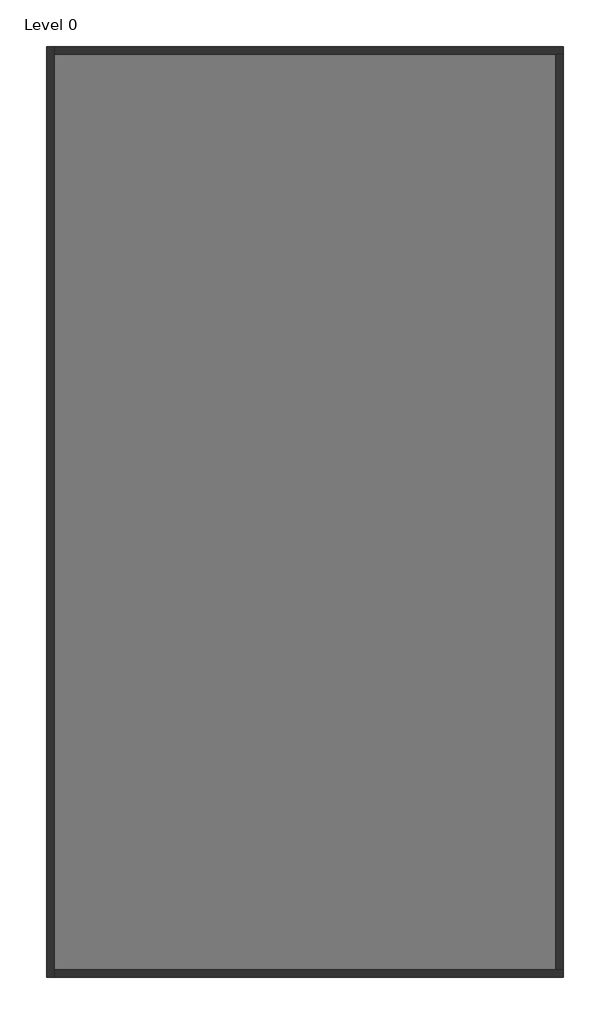
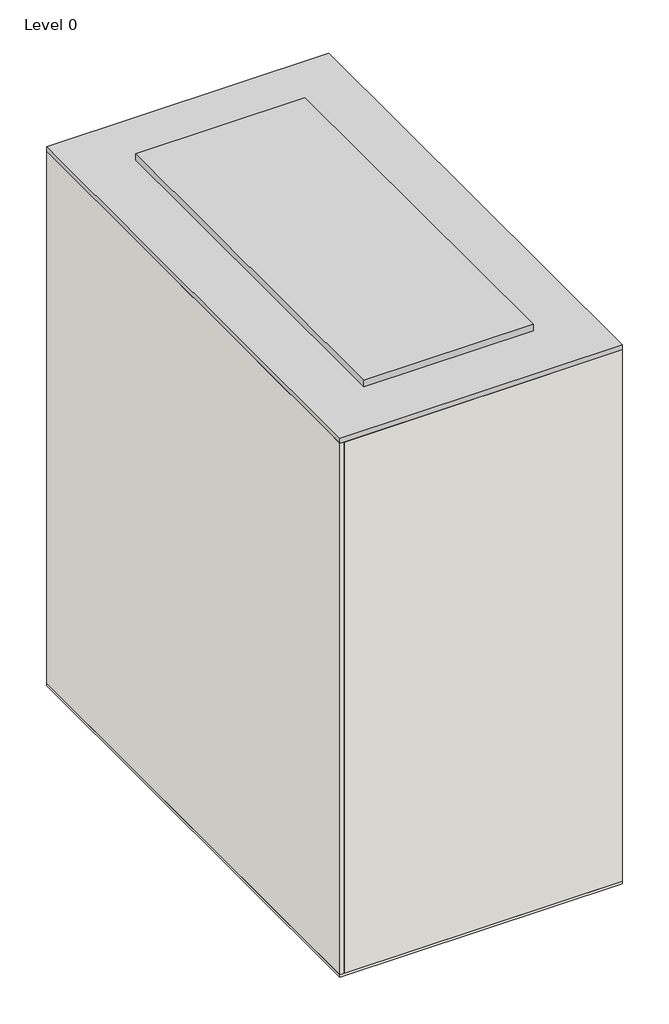
# One storey: 4 walls, 1 proxy, 1 slab.
"""IFC4 building model written with IfcOpenShell, lengths in millimetres."""

import ifcopenshell
import ifcopenshell.guid

model = None  # the IFC model being written
_history = None  # IfcOwnerHistory: only IFC2X3 demands one
_inside = {}  # id of a spatial element -> (the spatial element, [elements in it])
_under = {}  # id of a project, library or spatial element -> (it, [spatial elements below it])
_declared = {}  # id of a project -> (the project, [libraries it declares])
_typed = {}  # id of a type object -> (the type object, [elements of that type])
_made_of = {}  # id of a material, layer set ... -> (it, [elements and type objects made of it])


def new_model(schema):
    """Start an empty IFC model of exactly this schema.

    Asked for "IFC4X3", IfcOpenShell would pick the latest addendum, in which some entities
    have other attributes; the version numbers below select the first issue.
    IFC2X3 requires an IfcOwnerHistory on every rooted entity: one is made here for all.
    """
    global model, _history
    if schema == "IFC4X3":
        model = ifcopenshell.file(schema_version=(4, 3, 0, 0))
    else:
        model = ifcopenshell.file(schema=schema)
    _inside.clear()
    _under.clear()
    _declared.clear()
    _typed.clear()
    _made_of.clear()
    _history = None
    if model.schema == "IFC2X3":
        org = make("IfcOrganization", Name="unknown")
        user = make(
            "IfcPersonAndOrganization",
            ThePerson=make("IfcPerson", FamilyName="unknown"),
            TheOrganization=org,
        )
        app = make(
            "IfcApplication",
            ApplicationDeveloper=org,
            Version="unknown",
            ApplicationFullName="unknown",
            ApplicationIdentifier="unknown",
        )
        _history = make(
            "IfcOwnerHistory",
            OwningUser=user,
            OwningApplication=app,
            ChangeAction="ADDED",
            CreationDate=0,
        )
    return model


def make(cls, **values):
    """One entity of the class cls with the attributes given. An attribute that is None is left unset."""
    return model.create_entity(
        cls, **{name: value for name, value in values.items() if value is not None}
    )


def rooted(cls, **values):
    """An entity with a GlobalId (a new one), such as an element, a storey or a relation."""
    return make(cls, GlobalId=ifcopenshell.guid.new(), OwnerHistory=_history, **values)


def si_unit(unit_type, name, prefix=None):
    """IfcSIUnit, for example si_unit("LENGTHUNIT", "METRE", prefix="MILLI")."""
    return make("IfcSIUnit", UnitType=unit_type, Prefix=prefix, Name=name)


def assignment(units):
    """IfcUnitAssignment: the units of a project."""
    return None if units is None else make("IfcUnitAssignment", Units=units)


def point(xyz):
    """IfcCartesianPoint."""
    return None if xyz is None else make("IfcCartesianPoint", Coordinates=xyz)


def direction(xyz):
    """IfcDirection."""
    return None if xyz is None else make("IfcDirection", DirectionRatios=xyz)


def frame(location, z_axis=None, x_axis=None):
    """IfcAxis2Placement3D, a coordinate frame: its origin and axes. An axis left out is left unset."""
    return make(
        "IfcAxis2Placement3D",
        Location=point(location),
        Axis=direction(z_axis),
        RefDirection=direction(x_axis),
    )


def origin():
    """The frame at (0, 0, 0) with its axes left unset."""
    return frame((0.0, 0.0, 0.0))


def origin_with_axes():
    """The frame at (0, 0, 0) with the z axis (0, 0, 1) and the x axis (1, 0, 0) written out."""
    return frame((0.0, 0.0, 0.0), z_axis=(0.0, 0.0, 1.0), x_axis=(1.0, 0.0, 0.0))


def place(relative_to, where):
    """IfcLocalPlacement: puts the frame where relative to a parent placement (None: the world)."""
    return make(
        "IfcLocalPlacement", PlacementRelTo=relative_to, RelativePlacement=where
    )


def context(
    kind, dimensions, precision=None, world=None, true_north=None, identifier=None
):
    """IfcGeometricRepresentationContext, for example the 3D "Model" context."""
    return make(
        "IfcGeometricRepresentationContext",
        ContextIdentifier=identifier,
        ContextType=kind,
        CoordinateSpaceDimension=dimensions,
        Precision=precision,
        WorldCoordinateSystem=world,
        TrueNorth=true_north,
    )


def project(units=None, contexts=None):
    """IfcProject with its units and contexts."""
    return rooted(
        "IfcProject",
        Name="project",
        RepresentationContexts=contexts,
        UnitsInContext=assignment(units),
    )


def spatial(cls, under=None, at=None, **own):
    """A site, building, storey or space (cls), placed at a placement, below another one or the project."""
    s = rooted(cls, ObjectPlacement=at, **own)
    if under is not None:
        _under.setdefault(under.id(), (under, []))[1].append(s)
    return s


def polyline(points):
    """IfcPolyline through the points."""
    return make("IfcPolyline", Points=[point(p) for p in points])


def outline(outer, holes=None, kind="AREA"):
    """IfcArbitraryClosedProfileDef: a profile drawn as a closed curve; with holes, ...WithVoids."""
    if holes is None:
        return make("IfcArbitraryClosedProfileDef", ProfileType=kind, OuterCurve=outer)
    return make(
        "IfcArbitraryProfileDefWithVoids",
        ProfileType=kind,
        OuterCurve=outer,
        InnerCurves=holes,
    )


def extrude(swept, where, along, depth):
    """IfcExtrudedAreaSolid: the profile swept, set in the frame where, extruded along a direction by depth."""
    return make(
        "IfcExtrudedAreaSolid",
        SweptArea=swept,
        Position=where,
        ExtrudedDirection=direction(along),
        Depth=depth,
    )


def faces_of(points, faces, orient=None, outer=None):
    """IfcFace entities. A face is a list of loops; a loop is a list of indices into points, from 0.

    orient and outer hold one flag for each loop. By default every Orientation is true, the
    first loop of a face is its IfcFaceOuterBound and the others are IfcFaceBound.
    """
    made = []
    for i, loops in enumerate(faces):
        bounds = []
        for j, loop in enumerate(loops):
            is_outer = j == 0 if outer is None else outer[i][j]
            bounds.append(
                make(
                    "IfcFaceOuterBound" if is_outer else "IfcFaceBound",
                    Bound=make("IfcPolyLoop", Polygon=[points[k] for k in loop]),
                    Orientation=True if orient is None else orient[i][j],
                )
            )
        made.append(make("IfcFace", Bounds=bounds))
    return made


def faceted_brep(points, faces, orient=None, outer=None, voids=None):
    """IfcFacetedBrep: a solid bounded by flat faces; with voids (closed shells), ...WithVoids."""
    shared = [point(p) for p in points]
    hull = make("IfcClosedShell", CfsFaces=faces_of(shared, faces, orient, outer))
    if voids is None:
        return make("IfcFacetedBrep", Outer=hull)
    return make(
        "IfcFacetedBrepWithVoids",
        Outer=hull,
        Voids=[
            make(cls, CfsFaces=faces_of(shared, fs, o, b)) for cls, fs, o, b in voids
        ],
    )


def shape(context_of_items, identifier, shape_type, items):
    """IfcShapeRepresentation: the items that make up one representation, for example the "Body"."""
    return make(
        "IfcShapeRepresentation",
        ContextOfItems=context_of_items,
        RepresentationIdentifier=identifier,
        RepresentationType=shape_type,
        Items=items,
    )


def made_of(thing, what):
    """Note that an element or type object is made of a material, layer set ...; save() writes the relation."""
    if what is not None:
        _made_of.setdefault(what.id(), (what, []))[1].append(thing)
    return thing


def element(
    cls,
    number,
    at=None,
    inside=None,
    cuts=None,
    type_object=None,
    material=None,
    context=None,
    identifier="Body",
    shape_type=None,
    held_by="IfcProductDefinitionShape",
    body=None,
    shapes=None,
    **own,
):
    """One element of the class cls, such as IfcWall. Its Tag is "e" and its number.

    at: its placement. inside: the storey or other place that contains it. cuts: it is an
    opening in that element (IfcRelVoidsElement). A single representation is given by context,
    identifier, shape_type and body (its items); several are given by shapes. held_by: the class
    of the entity that holds the representations. save() writes the other relations.
    """
    e = rooted(cls, Tag="e%d" % number, ObjectPlacement=at, **own)
    if body is not None:
        shapes = [shape(context, identifier, shape_type, body)]
    if shapes is not None:
        e.Representation = make(held_by, Representations=shapes)
    if inside is not None:
        _inside.setdefault(inside.id(), (inside, []))[1].append(e)
    if cuts is not None:
        rooted(
            "IfcRelVoidsElement", RelatingBuildingElement=cuts, RelatedOpeningElement=e
        )
    if type_object is not None:
        _typed.setdefault(type_object.id(), (type_object, []))[1].append(e)
    return made_of(e, material)


def aggregate(whole, parts):
    """IfcRelAggregates: a whole, such as a stair, and the parts it consists of."""
    return rooted("IfcRelAggregates", RelatingObject=whole, RelatedObjects=parts)


def save(model, path):
    """Write the relations noted so far, then the file.

    IfcRelAggregates (storeys below a building ...), IfcRelContainedInSpatialStructure (elements
    in a storey), IfcRelDefinesByType, IfcRelAssociatesMaterial and IfcRelDeclares: one each for
    every whole, place, type object, material and project.
    """
    for whole, parts in _under.values():
        aggregate(whole, parts)
    for where, things in _inside.values():
        rooted(
            "IfcRelContainedInSpatialStructure",
            RelatedElements=things,
            RelatingStructure=where,
        )
    for kind, things in _typed.values():
        rooted("IfcRelDefinesByType", RelatedObjects=things, RelatingType=kind)
    for what, things in _made_of.values():
        rooted("IfcRelAssociatesMaterial", RelatedObjects=things, RelatingMaterial=what)
    for by, libraries in _declared.values():
        rooted("IfcRelDeclares", RelatingContext=by, RelatedDefinitions=libraries)
    model.write(path)


model = new_model("IFC4")

# Units and contexts
model_context = context("Model", 3, world=origin())
ifc_project = project(units=[si_unit("LENGTHUNIT", "METRE", prefix="MILLI")], contexts=[model_context])

# Site, building, storey
site = spatial("IfcSite", under=ifc_project)
building = spatial("IfcBuilding", under=site)
storey = spatial("IfcBuildingStorey", under=building, Name="Level 0", Elevation=100.0)

# Proxy
placement = place(None, origin())
element("IfcBuildingElementProxy", 1, Name="LowUrbanDensityBuilding : LowUrbanDensityBuilding", ObjectType="LowUrbanDensityBuilding : LowUrbanDensityBuilding", at=placement, inside=storey, context=model_context, shape_type="SweptSolid", body=[
    extrude(outline(polyline([(7325.2659446, 3676.2074539), (7325.2659446, -14323.7925461), (-2674.7340554, -14323.7925461), (-2674.7340554, 3676.2074539), (7325.2659446, 3676.2074539)])), origin_with_axes(), (0.0, 0.0, 1.0), 20200.0),
    extrude(outline(polyline([(5325.2659446, 1676.2074539), (5325.2659446, -12323.7925461), (-674.7340554, -12323.7925461), (-674.7340554, 1676.2074539), (5325.2659446, 1676.2074539)])), frame((0.0, 0.0, 20200.0), z_axis=(0.0, 0.0, 1.0), x_axis=(1.0, 0.0, 0.0)), (0.0, 0.0, 1.0), 245.0),
])

# Slab
element("IfcSlab", 2, ObjectType="Floor-Concrete_100Con", at=placement, inside=storey, context=model_context, shape_type="SweptSolid", body=[
    extrude(outline(polyline([(7325.2659446, 3676.2074539), (7325.2659446, -14323.7925461), (-2674.7340554, -14323.7925461), (-2674.7340554, 3676.2074539), (7325.2659446, 3676.2074539)])), origin_with_axes(), (0.0, 0.0, 1.0), 100.0),
])

# Walls
element("IfcWall", 3, ObjectType="Wall-Ext_25Rdr-100Blk-19P", at=placement, inside=storey, context=model_context, shape_type="Brep", body=[
    faceted_brep([(-2674.7340554, 3676.2074539, 100.0), (-2674.7340554, -14323.7925461, 100.0), (-2674.7340554, -14323.7925461, 20000.0), (-2674.7340554, 3676.2074539, 20000.0), (-2530.4340554, 3676.2074539, 100.0), (-2530.4340554, 3676.2074539, 20000.0), (-2530.4340554, 3531.9074539, 20000.0), (-2530.4340554, -14179.4925461, 20000.0), (-2530.4340554, -14323.7925461, 20000.0), (-2530.4340554, -14323.7925461, 100.0), (-2530.4340554, -14179.4925461, 100.0), (-2530.4340554, 3531.9074539, 100.0)], [[[0, 1, 2, 3]], [[4, 5, 6, 7, 8, 9, 10, 11]], [[1, 0, 4, 11, 10, 9]], [[3, 2, 8, 7, 6, 5]], [[2, 1, 9, 8]], [[0, 3, 5, 4]]]),
])
element("IfcWall", 4, ObjectType="Wall-Ext_25Rdr-100Blk-19P", at=placement, inside=storey, context=model_context, shape_type="Brep", body=[
    faceted_brep([(-2530.4340554, -14323.7925461, 100.0), (7325.2659446, -14323.7925461, 100.0), (7325.2659446, -14323.7925461, 20000.0), (-2530.4340554, -14323.7925461, 20000.0), (-2530.4340554, -14179.4925461, 100.0), (-2530.4340554, -14179.4925461, 20000.0), (7180.9659446, -14179.4925461, 20000.0), (7325.2659446, -14179.4925461, 20000.0), (7325.2659446, -14179.4925461, 100.0), (7180.9659446, -14179.4925461, 100.0)], [[[0, 1, 2, 3]], [[4, 5, 6, 7, 8, 9]], [[1, 0, 4, 9, 8]], [[3, 2, 7, 6, 5]], [[0, 3, 5, 4]], [[2, 1, 8, 7]]]),
])
element("IfcWall", 5, ObjectType="Wall-Ext_25Rdr-100Blk-19P", at=placement, inside=storey, context=model_context, shape_type="Brep", body=[
    faceted_brep([(7325.2659446, 3676.2074539, 100.0), (-2530.4340554, 3676.2074539, 100.0), (-2530.4340554, 3676.2074539, 20000.0), (7325.2659446, 3676.2074539, 20000.0), (7325.2659446, 3531.9074539, 100.0), (7325.2659446, 3531.9074539, 20000.0), (7180.9659446, 3531.9074539, 20000.0), (-2530.4340554, 3531.9074539, 20000.0), (-2530.4340554, 3531.9074539, 100.0), (7180.9659446, 3531.9074539, 100.0)], [[[0, 1, 2, 3]], [[4, 5, 6, 7, 8, 9]], [[1, 0, 4, 9, 8]], [[3, 2, 7, 6, 5]], [[2, 1, 8, 7]], [[0, 3, 5, 4]]]),
])
element("IfcWall", 6, ObjectType="Wall-Ext_25Rdr-100Blk-19P", at=placement, inside=storey, context=model_context, shape_type="SweptSolid", body=[
    extrude(outline(polyline([(7325.2659446, 3531.9074539), (7325.2659446, -14179.4925461), (7180.9659446, -14179.4925461), (7180.9659446, 3531.9074539), (7325.2659446, 3531.9074539)])), frame((0.0, 0.0, 100.0), z_axis=(0.0, 0.0, 1.0), x_axis=(1.0, 0.0, 0.0)), (0.0, 0.0, 1.0), 19900.0),
])

save(model, "model.ifc")

# Revit data of these elements
# Project information
#   Project Issue Date = "Issue Date"
#   Project Status = "Project Status"
#   Client Name = "Owner"
#   Project Address = "Enter address here"
#   Project Name = "Project Name"
#   Project Number = "Project Number"
# Type "Floor-Concrete_100Con"
#   Keynote = "E60/130"
#   Function = 0
#   Layers, outside or top first: 100 mm "Concrete" (function 1)
# Type "Wall-Ext_25Rdr-100Blk-19P"
#   Keynote = "F10"
#   Layers, outside or top first: 25.3 mm "Render, Beige, Smooth" (function 5); 100 mm "Concrete Masonry Units _Low Density" (function 1); 19 mm "Plaster" (function 5)
# Element 1 (IfcBuildingElementProxy, "LowUrbanDensityBuilding : LowUrbanDensityBuilding")
#   Phase Created = New Construction
#   Materials on its faces: "Default Form"
# Element 2 (IfcSlab, "Floor-Concrete_100Con")
#   Height Offset From Level = 0 mm
#   Phase Created = New Construction
#   Materials on its faces: "Concrete"
# Element 3 (IfcWall, "Wall-Ext_25Rdr-100Blk-19P")
#   Top Offset = 0 mm
#   Base Offset = 0 mm
#   wall height = 19900 mm
#   Phase Created = New Construction
#   Base Constraint = Level 0
#   Top Constraint = Level 5
#   Materials on its faces: "Render, Beige, Smooth", "Default Wall", "Plaster"
# Elements 4, 5, 6 (IfcWall, "Wall-Ext_25Rdr-100Blk-19P")
#   Top Offset = 0 mm
#   Base Offset = 0 mm
#   wall height = 19900 mm
#   Phase Created = New Construction
#   Base Constraint = Level 0
#   Top Constraint = Level 5
#   Materials on its faces: "Default Wall", "Render, Beige, Smooth", "Plaster"
# Materials
#   "Concrete": class "Concrete", colour RGB 120 120 120, transparency 0, Description = "Portland Cement Concrete", Cost = 0
#   "Render, Beige, Smooth": class "Generic", colour RGB 213 198 180, transparency 0, Description = "physical material", Cost = 0
#   "Concrete Masonry Units _Low Density": class "Masonry", colour RGB 181 181 181, transparency 0, Description = "Concrete masonry units", Cost = 0
#   "Plaster": class "Generic", colour RGB 249 249 249, transparency 0, Description = "Plaster", Cost = 0
#   "Default Form": class "Generic", colour RGB 185 189 196, transparency 0.5, Cost = 0
#   "Default Wall": class "Miscellaneous", colour RGB 128 128 128, transparency 0, Comments = "Rendering appearance not upgraded Rendering appearance not upgraded ", Cost = 0
